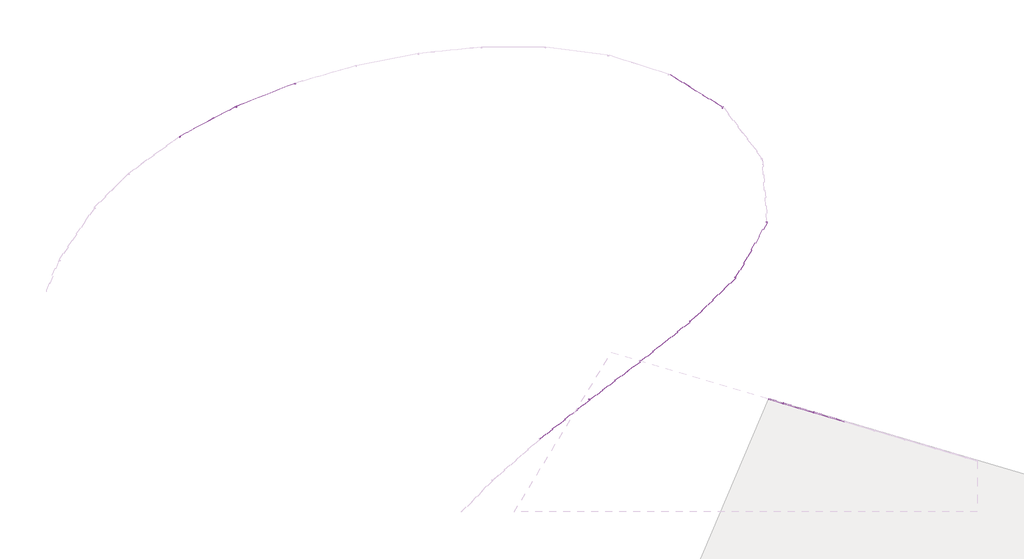
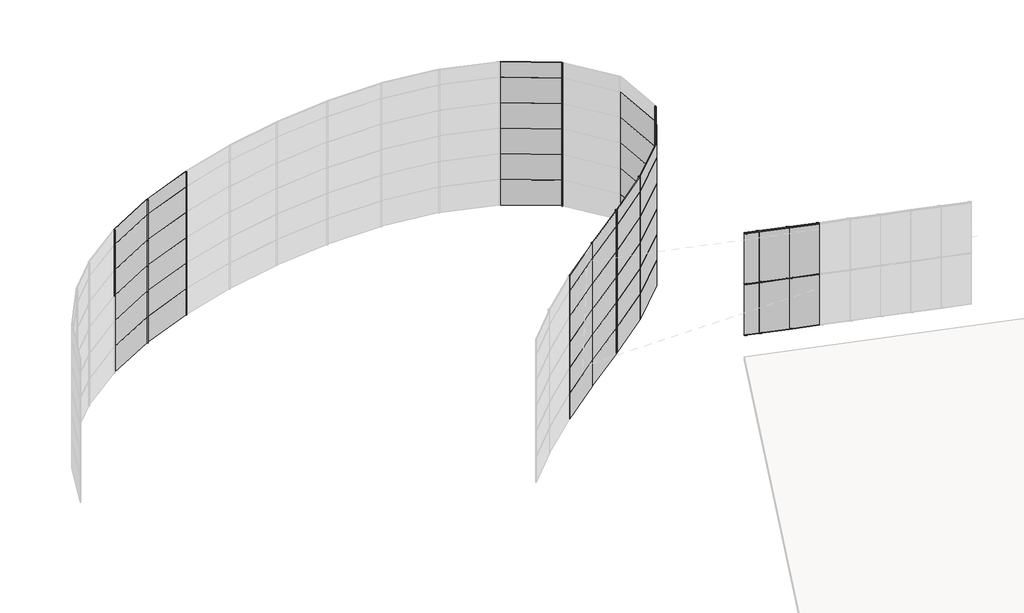
# One storey, part 6 of 8: 60 members, 59 plates.
"""IFC4 building model written with IfcOpenShell, lengths in millimetres."""

import ifcopenshell
import ifcopenshell.guid

model = None  # the IFC model being written
_history = None  # IfcOwnerHistory: only IFC2X3 demands one
_inside = {}  # id of a spatial element -> (the spatial element, [elements in it])
_under = {}  # id of a project, library or spatial element -> (it, [spatial elements below it])
_declared = {}  # id of a project -> (the project, [libraries it declares])
_typed = {}  # id of a type object -> (the type object, [elements of that type])
_made_of = {}  # id of a material, layer set ... -> (it, [elements and type objects made of it])


def new_model(schema):
    """Start an empty IFC model of exactly this schema.

    Asked for "IFC4X3", IfcOpenShell would pick the latest addendum, in which some entities
    have other attributes; the version numbers below select the first issue.
    IFC2X3 requires an IfcOwnerHistory on every rooted entity: one is made here for all.
    """
    global model, _history
    if schema == "IFC4X3":
        model = ifcopenshell.file(schema_version=(4, 3, 0, 0))
    else:
        model = ifcopenshell.file(schema=schema)
    _inside.clear()
    _under.clear()
    _declared.clear()
    _typed.clear()
    _made_of.clear()
    _history = None
    if model.schema == "IFC2X3":
        org = make("IfcOrganization", Name="unknown")
        user = make(
            "IfcPersonAndOrganization",
            ThePerson=make("IfcPerson", FamilyName="unknown"),
            TheOrganization=org,
        )
        app = make(
            "IfcApplication",
            ApplicationDeveloper=org,
            Version="unknown",
            ApplicationFullName="unknown",
            ApplicationIdentifier="unknown",
        )
        _history = make(
            "IfcOwnerHistory",
            OwningUser=user,
            OwningApplication=app,
            ChangeAction="ADDED",
            CreationDate=0,
        )
    return model


def make(cls, **values):
    """One entity of the class cls with the attributes given. An attribute that is None is left unset."""
    return model.create_entity(
        cls, **{name: value for name, value in values.items() if value is not None}
    )


def rooted(cls, **values):
    """An entity with a GlobalId (a new one), such as an element, a storey or a relation."""
    return make(cls, GlobalId=ifcopenshell.guid.new(), OwnerHistory=_history, **values)


def si_unit(unit_type, name, prefix=None):
    """IfcSIUnit, for example si_unit("LENGTHUNIT", "METRE", prefix="MILLI")."""
    return make("IfcSIUnit", UnitType=unit_type, Prefix=prefix, Name=name)


def assignment(units):
    """IfcUnitAssignment: the units of a project."""
    return None if units is None else make("IfcUnitAssignment", Units=units)


def point(xyz):
    """IfcCartesianPoint."""
    return None if xyz is None else make("IfcCartesianPoint", Coordinates=xyz)


def direction(xyz):
    """IfcDirection."""
    return None if xyz is None else make("IfcDirection", DirectionRatios=xyz)


def frame(location, z_axis=None, x_axis=None):
    """IfcAxis2Placement3D, a coordinate frame: its origin and axes. An axis left out is left unset."""
    return make(
        "IfcAxis2Placement3D",
        Location=point(location),
        Axis=direction(z_axis),
        RefDirection=direction(x_axis),
    )


def frame_2d(location, x_axis=None):
    """IfcAxis2Placement2D, a coordinate frame in the plane: its origin and x axis."""
    return make(
        "IfcAxis2Placement2D", Location=point(location), RefDirection=direction(x_axis)
    )


def origin():
    """The frame at (0, 0, 0) with its axes left unset."""
    return frame((0.0, 0.0, 0.0))


def origin_with_axes():
    """The frame at (0, 0, 0) with the z axis (0, 0, 1) and the x axis (1, 0, 0) written out."""
    return frame((0.0, 0.0, 0.0), z_axis=(0.0, 0.0, 1.0), x_axis=(1.0, 0.0, 0.0))


def origin_2d():
    """The frame at (0, 0) in the plane with its x axis left unset."""
    return frame_2d((0.0, 0.0))


def place(relative_to, where):
    """IfcLocalPlacement: puts the frame where relative to a parent placement (None: the world)."""
    return make(
        "IfcLocalPlacement", PlacementRelTo=relative_to, RelativePlacement=where
    )


def context(
    kind, dimensions, precision=None, world=None, true_north=None, identifier=None
):
    """IfcGeometricRepresentationContext, for example the 3D "Model" context."""
    return make(
        "IfcGeometricRepresentationContext",
        ContextIdentifier=identifier,
        ContextType=kind,
        CoordinateSpaceDimension=dimensions,
        Precision=precision,
        WorldCoordinateSystem=world,
        TrueNorth=true_north,
    )


def project(units=None, contexts=None):
    """IfcProject with its units and contexts."""
    return rooted(
        "IfcProject",
        Name="project",
        RepresentationContexts=contexts,
        UnitsInContext=assignment(units),
    )


def spatial(cls, under=None, at=None, **own):
    """A site, building, storey or space (cls), placed at a placement, below another one or the project."""
    s = rooted(cls, ObjectPlacement=at, **own)
    if under is not None:
        _under.setdefault(under.id(), (under, []))[1].append(s)
    return s


def polyline(points):
    """IfcPolyline through the points."""
    return make("IfcPolyline", Points=[point(p) for p in points])


def circle_curve(where, radius):
    """IfcCircle in the frame where."""
    return make("IfcCircle", Position=where, Radius=radius)


def trimmed(basis, trim1, trim2, sense, master):
    """IfcTrimmedCurve: the piece of a basis curve between two trims."""
    return make(
        "IfcTrimmedCurve",
        BasisCurve=basis,
        Trim1=trim1,
        Trim2=trim2,
        SenseAgreement=sense,
        MasterRepresentation=master,
    )


def segment(curve, same_sense, transition):
    """IfcCompositeCurveSegment."""
    return make(
        "IfcCompositeCurveSegment",
        Transition=transition,
        SameSense=same_sense,
        ParentCurve=curve,
    )


def composite_curve(segments, self_intersect=None):
    """IfcCompositeCurve: segments joined end to end."""
    return make("IfcCompositeCurve", Segments=segments, SelfIntersect=self_intersect)


def outline(outer, holes=None, kind="AREA"):
    """IfcArbitraryClosedProfileDef: a profile drawn as a closed curve; with holes, ...WithVoids."""
    if holes is None:
        return make("IfcArbitraryClosedProfileDef", ProfileType=kind, OuterCurve=outer)
    return make(
        "IfcArbitraryProfileDefWithVoids",
        ProfileType=kind,
        OuterCurve=outer,
        InnerCurves=holes,
    )


def extrude(swept, where, along, depth):
    """IfcExtrudedAreaSolid: the profile swept, set in the frame where, extruded along a direction by depth."""
    return make(
        "IfcExtrudedAreaSolid",
        SweptArea=swept,
        Position=where,
        ExtrudedDirection=direction(along),
        Depth=depth,
    )


def shape(context_of_items, identifier, shape_type, items):
    """IfcShapeRepresentation: the items that make up one representation, for example the "Body"."""
    return make(
        "IfcShapeRepresentation",
        ContextOfItems=context_of_items,
        RepresentationIdentifier=identifier,
        RepresentationType=shape_type,
        Items=items,
    )


def source(mapping_origin, context_of_items, identifier, shape_type, items):
    """IfcRepresentationMap: a shape defined once, which mapped items show again and again."""
    return make(
        "IfcRepresentationMap",
        MappingOrigin=mapping_origin,
        MappedRepresentation=shape(context_of_items, identifier, shape_type, items),
    )


def transform(
    local_origin,
    x_axis=None,
    y_axis=None,
    z_axis=None,
    scale=None,
    scale2=None,
    scale3=None,
    uniform=True,
):
    """IfcCartesianTransformationOperator3D, or its non-uniform kind. x_axis, y_axis, z_axis: its Axis1, 2, 3."""
    if uniform:
        return make(
            "IfcCartesianTransformationOperator3D",
            Axis1=direction(x_axis),
            Axis2=direction(y_axis),
            LocalOrigin=point(local_origin),
            Scale=scale,
            Axis3=direction(z_axis),
        )
    return make(
        "IfcCartesianTransformationOperator3DnonUniform",
        Axis1=direction(x_axis),
        Axis2=direction(y_axis),
        LocalOrigin=point(local_origin),
        Scale=scale,
        Axis3=direction(z_axis),
        Scale2=scale2,
        Scale3=scale3,
    )


def mapped(mapping_source, mapping_target):
    """IfcMappedItem: shows the shape of a source again, moved by a transform."""
    return make(
        "IfcMappedItem", MappingSource=mapping_source, MappingTarget=mapping_target
    )


def made_of(thing, what):
    """Note that an element or type object is made of a material, layer set ...; save() writes the relation."""
    if what is not None:
        _made_of.setdefault(what.id(), (what, []))[1].append(thing)
    return thing


def element(
    cls,
    number,
    at=None,
    inside=None,
    cuts=None,
    type_object=None,
    material=None,
    context=None,
    identifier="Body",
    shape_type=None,
    held_by="IfcProductDefinitionShape",
    body=None,
    shapes=None,
    **own,
):
    """One element of the class cls, such as IfcWall. Its Tag is "e" and its number.

    at: its placement. inside: the storey or other place that contains it. cuts: it is an
    opening in that element (IfcRelVoidsElement). A single representation is given by context,
    identifier, shape_type and body (its items); several are given by shapes. held_by: the class
    of the entity that holds the representations. save() writes the other relations.
    """
    e = rooted(cls, Tag="e%d" % number, ObjectPlacement=at, **own)
    if body is not None:
        shapes = [shape(context, identifier, shape_type, body)]
    if shapes is not None:
        e.Representation = make(held_by, Representations=shapes)
    if inside is not None:
        _inside.setdefault(inside.id(), (inside, []))[1].append(e)
    if cuts is not None:
        rooted(
            "IfcRelVoidsElement", RelatingBuildingElement=cuts, RelatedOpeningElement=e
        )
    if type_object is not None:
        _typed.setdefault(type_object.id(), (type_object, []))[1].append(e)
    return made_of(e, material)


def aggregate(whole, parts):
    """IfcRelAggregates: a whole, such as a stair, and the parts it consists of."""
    return rooted("IfcRelAggregates", RelatingObject=whole, RelatedObjects=parts)


def save(model, path):
    """Write the relations noted so far, then the file.

    IfcRelAggregates (storeys below a building ...), IfcRelContainedInSpatialStructure (elements
    in a storey), IfcRelDefinesByType, IfcRelAssociatesMaterial and IfcRelDeclares: one each for
    every whole, place, type object, material and project.
    """
    for whole, parts in _under.values():
        aggregate(whole, parts)
    for where, things in _inside.values():
        rooted(
            "IfcRelContainedInSpatialStructure",
            RelatedElements=things,
            RelatingStructure=where,
        )
    for kind, things in _typed.values():
        rooted("IfcRelDefinesByType", RelatedObjects=things, RelatingType=kind)
    for what, things in _made_of.values():
        rooted("IfcRelAssociatesMaterial", RelatedObjects=things, RelatingMaterial=what)
    for by, libraries in _declared.values():
        rooted("IfcRelDeclares", RelatingContext=by, RelatedDefinitions=libraries)
    model.write(path)


def montante_circular_25_mm_raio_ce826986(model_context):
    return source(origin(), model_context, "Body", "SweptSolid", [
        extrude(outline(composite_curve([segment(trimmed(circle_curve(frame_2d((-25.0, 0.0)), 25.0), [point((0.0, 0.0))], [point((-50.0, 0.0))], False, "CARTESIAN"), True, "CONTINUOUS"), segment(trimmed(circle_curve(frame_2d((-25.0, 0.0)), 25.0), [point((-50.0, 0.0))], [point((0.0, 0.0))], False, "CARTESIAN"), True, "CONTINUOUS")], self_intersect=False)), frame((0.0, 0.0, -1500.0), z_axis=(0.0, 0.0, 1.0), x_axis=(1.0, 0.0, 0.0)), (0.0, 0.0, 1.0), 1500.0),
    ])


def montante_circular_25_mm_raio_36e581cf(model_context):
    return source(origin(), model_context, "Body", "SweptSolid", [
        extrude(outline(composite_curve([segment(trimmed(circle_curve(origin_2d(), 25.0), [point((25.0, 0.0))], [point((-25.0, 0.0))], False, "CARTESIAN"), True, "CONTINUOUS"), segment(trimmed(circle_curve(origin_2d(), 25.0), [point((-25.0, 0.0))], [point((25.0, 0.0))], False, "CARTESIAN"), True, "CONTINUOUS")], self_intersect=False)), frame((0.0, 0.0, -1500.0), z_axis=(0.0, 0.0, 1.0), x_axis=(1.0, 0.0, 0.0)), (0.0, 0.0, 1.0), 1500.0),
    ])


def montante_circular_25_mm_raio_f24612f6(model_context):
    return source(origin(), model_context, "Body", "SweptSolid", [
        extrude(outline(composite_curve([segment(trimmed(circle_curve(frame_2d((-25.0, 0.0)), 25.0), [point((0.0, 0.0))], [point((-50.0, 0.0))], False, "CARTESIAN"), True, "CONTINUOUS"), segment(trimmed(circle_curve(frame_2d((-25.0, 0.0)), 25.0), [point((-50.0, 0.0))], [point((0.0, 0.0))], False, "CARTESIAN"), True, "CONTINUOUS")], self_intersect=False)), frame((0.0, 0.0, -727.4383788), z_axis=(0.0, 0.0, 1.0), x_axis=(1.0, 0.0, 0.0)), (0.0, 0.0, 1.0), 727.4383788),
    ])


def montante_circular_25_mm_raio_a1f35a82(model_context):
    return source(origin(), model_context, "Body", "SweptSolid", [
        extrude(outline(composite_curve([segment(trimmed(circle_curve(origin_2d(), 25.0), [point((25.0, 0.0))], [point((-25.0, 0.0))], False, "CARTESIAN"), True, "CONTINUOUS"), segment(trimmed(circle_curve(origin_2d(), 25.0), [point((-25.0, 0.0))], [point((25.0, 0.0))], False, "CARTESIAN"), True, "CONTINUOUS")], self_intersect=False)), frame((0.0, 0.0, -727.4383788), z_axis=(0.0, 0.0, 1.0), x_axis=(1.0, 0.0, 0.0)), (0.0, 0.0, 1.0), 727.4383788),
    ])


def montante_circular_25_mm_raio_8ba79aec(model_context):
    return source(origin(), model_context, "Body", "SweptSolid", [
        extrude(outline(composite_curve([segment(trimmed(circle_curve(origin_2d(), 25.0), [point((25.0, 0.0))], [point((-25.0, 0.0))], False, "CARTESIAN"), True, "CONTINUOUS"), segment(trimmed(circle_curve(origin_2d(), 25.0), [point((-25.0, 0.0))], [point((25.0, 0.0))], False, "CARTESIAN"), True, "CONTINUOUS")], self_intersect=False)), frame((0.0, 0.0, -900.0), z_axis=(0.0, 0.0, 1.0), x_axis=(1.0, 0.0, 0.0)), (0.0, 0.0, 1.0), 900.0),
    ])


def painel_do_sistema_5ef9eced(model_context):
    return source(origin(), model_context, "Body", "SweptSolid", [
        extrude(outline(polyline([(1475.0, 24.5), (-1475.0, 24.5), (-1475.0, 49.5), (1475.0, 49.5), (1475.0, 24.5)])), origin_with_axes(), (0.0, 0.0, 1.0), 1500.0),
    ])


def painel_do_sistema_bf426e09(model_context):
    return source(origin(), model_context, "Body", "SweptSolid", [
        extrude(outline(polyline([(1475.0, 24.5), (-1475.0, 24.5), (-1475.0, 49.5), (1475.0, 49.5), (1475.0, 24.5)])), origin_with_axes(), (0.0, 0.0, 1.0), 727.4383788),
    ])


def painel_do_sistema_85ccde5d(model_context):
    return source(origin(), model_context, "Body", "SweptSolid", [
        extrude(outline(polyline([(1475.0, -49.5), (-1475.0, -49.5), (-1475.0, -24.5), (1475.0, -24.5), (1475.0, -49.5)])), origin_with_axes(), (0.0, 0.0, 1.0), 1500.0),
    ])


def painel_do_sistema_d8fd150b(model_context):
    return source(origin(), model_context, "Body", "SweptSolid", [
        extrude(outline(polyline([(1475.0, -49.5), (-1475.0, -49.5), (-1475.0, -24.5), (1475.0, -24.5), (1475.0, -49.5)])), origin_with_axes(), (0.0, 0.0, 1.0), 900.0),
    ])


def painel_do_sistema_af596b93(model_context):
    return source(origin(), model_context, "Body", "SweptSolid", [
        extrude(outline(polyline([(1462.4999925, 24.5), (-1462.4999925, 24.5), (-1462.4999925, 49.5), (1462.4999925, 49.5), (1462.4999925, 24.5)])), origin_with_axes(), (0.0, 0.0, 1.0), 1500.0),
    ])


def painel_do_sistema_44dfe8f0(model_context):
    return source(origin(), model_context, "Body", "SweptSolid", [
        extrude(outline(polyline([(1462.4999925, 24.5), (-1462.4999925, 24.5), (-1462.4999925, 49.5), (1462.4999925, 49.5), (1462.4999925, 24.5)])), origin_with_axes(), (0.0, 0.0, 1.0), 727.4383788),
    ])


model = new_model("IFC4")

# Units and contexts
model_context = context("Model", 3, world=origin())
ifc_project = project(units=[si_unit("LENGTHUNIT", "METRE", prefix="MILLI")], contexts=[model_context])

# Site, building, storey
site = spatial("IfcSite", under=ifc_project)
building = spatial("IfcBuilding", under=site)
storey = spatial("IfcBuildingStorey", under=building, Name="Nível 3", Elevation=7695.2)

# Members
placement = place(None, origin())
montante_circular_25_mm_raio_shape = montante_circular_25_mm_raio_ce826986(model_context)
element("IfcMember", 1, ObjectType="Montante circular : 25 mm Raio", at=placement, inside=storey, context=model_context, shape_type="MappedRepresentation", body=[
    mapped(montante_circular_25_mm_raio_shape, transform((-4389.7681283, 32366.1480949, 15000.0), x_axis=(0.0, 0.0, 1.0), y_axis=(0.28318378939534594, 0.95906566064253, 0.0), z_axis=(-0.95906566064253, 0.28318378939534594, 0.0))),
])
element("IfcMember", 2, ObjectType="Montante circular : 25 mm Raio", at=placement, inside=storey, context=model_context, shape_type="MappedRepresentation", body=[
    mapped(montante_circular_25_mm_raio_shape, transform((-5828.3666192, 32790.923779, 15000.0), x_axis=(0.0, 0.0, 1.0), y_axis=(0.283183789395347, 0.9590656606425296, 0.0), z_axis=(-0.9590656606425296, 0.283183789395347, 0.0))),
])
montante_circular_25_mm_raio_2_shape = montante_circular_25_mm_raio_36e581cf(model_context)
element("IfcMember", 3, ObjectType="Montante circular : 25 mm Raio", at=placement, inside=storey, context=model_context, shape_type="MappedRepresentation", body=[
    mapped(montante_circular_25_mm_raio_2_shape, transform((-4389.7681283, 32366.1480949, 9000.000015), x_axis=(0.0, 0.0, 1.0), y_axis=(0.28318378939534594, 0.95906566064253, 0.0), z_axis=(-0.95906566064253, 0.28318378939534594, 0.0))),
])
element("IfcMember", 4, ObjectType="Montante circular : 25 mm Raio", at=placement, inside=storey, context=model_context, shape_type="MappedRepresentation", body=[
    mapped(montante_circular_25_mm_raio_2_shape, transform((-5828.3666192, 32790.923779, 9000.000015), x_axis=(0.0, 0.0, 1.0), y_axis=(0.283183789395347, 0.9590656606425296, 0.0), z_axis=(-0.9590656606425296, 0.283183789395347, 0.0))),
])
element("IfcMember", 5, ObjectType="Montante circular : 25 mm Raio", at=placement, inside=storey, context=model_context, shape_type="MappedRepresentation", body=[
    mapped(montante_circular_25_mm_raio_2_shape, transform((-4389.7681283, 32366.1480949, 12000.000015), x_axis=(0.0, 0.0, 1.0), y_axis=(0.28318378939534855, 0.9590656606425292, 0.0), z_axis=(-0.9590656606425291, 0.2831837893953485, 0.0))),
])
element("IfcMember", 6, ObjectType="Montante circular : 25 mm Raio", at=placement, inside=storey, context=model_context, shape_type="MappedRepresentation", body=[
    mapped(montante_circular_25_mm_raio_2_shape, transform((-5828.3666192, 32790.923779, 12000.000015), x_axis=(0.0, 0.0, 1.0), y_axis=(0.283183789395347, 0.9590656606425296, 0.0), z_axis=(-0.9590656606425296, 0.283183789395347, 0.0))),
])
element("IfcMember", 7, ObjectType="Montante circular : 25 mm Raio", at=placement, inside=storey, context=model_context, shape_type="MappedRepresentation", body=[
    mapped(montante_circular_25_mm_raio_2_shape, transform((-14996.1891623, 32974.6356945, 9000.0), x_axis=(0.7952150611070873, 0.6063274747102028, 0.0), y_axis=(0.6063274747102028, -0.7952150611070873, 0.0), z_axis=(0.0, 0.0, -1.0))),
])
element("IfcMember", 8, ObjectType="Montante circular : 25 mm Raio", at=placement, inside=storey, context=model_context, shape_type="MappedRepresentation", body=[
    mapped(montante_circular_25_mm_raio_2_shape, transform((-12604.1298635, 34785.1749266, 9000.0), x_axis=(0.7953870623365296, 0.6061018240095187, 0.0), y_axis=(0.6061018240095187, -0.7953870623365296, 0.0), z_axis=(0.0, 0.0, -1.0))),
])
element("IfcMember", 9, ObjectType="Montante circular : 25 mm Raio", at=placement, inside=storey, context=model_context, shape_type="MappedRepresentation", body=[
    mapped(montante_circular_25_mm_raio_2_shape, transform((-10255.474771, 36651.6741247, 9000.0), x_axis=(0.7627263023971693, 0.6467214142361005, 0.0), y_axis=(0.6467214142361005, -0.7627263023971693, 0.0), z_axis=(0.0, 0.0, -1.0))),
])
element("IfcMember", 10, ObjectType="Montante circular : 25 mm Raio", at=placement, inside=storey, context=model_context, shape_type="MappedRepresentation", body=[
    mapped(montante_circular_25_mm_raio_2_shape, transform((-8101.871437, 38740.2125323, 9000.0), x_axis=(0.6490334571140042, 0.7607598645739956, 0.0), y_axis=(0.7607598645739956, -0.6490334571140042, 0.0), z_axis=(0.0, 0.0, -1.0))),
])
element("IfcMember", 11, ObjectType="Montante circular : 25 mm Raio", at=placement, inside=storey, context=model_context, shape_type="MappedRepresentation", body=[
    mapped(montante_circular_25_mm_raio_2_shape, transform((-6627.5874319, 41352.9671461, 9000.0), x_axis=(0.24827563424230142, 0.9686894287859154, 0.0), y_axis=(0.9686894287859154, -0.24827563424230142, 0.0), z_axis=(0.0, 0.0, -1.0))),
])
element("IfcMember", 12, ObjectType="Montante circular : 25 mm Raio", at=placement, inside=storey, context=model_context, shape_type="MappedRepresentation", body=[
    mapped(montante_circular_25_mm_raio_2_shape, transform((-8685.5307871, 46730.4667655, 9000.0), x_axis=(-0.7608105002607386, 0.6489741001711892, 0.0), y_axis=(0.6489741001711892, 0.7608105002607386, 0.0), z_axis=(0.0, 0.0, -1.0))),
])
element("IfcMember", 13, ObjectType="Montante circular : 25 mm Raio", at=placement, inside=storey, context=model_context, shape_type="MappedRepresentation", body=[
    mapped(montante_circular_25_mm_raio_2_shape, transform((-28892.5410808, 47874.3709699, 9000.0), x_axis=(-0.9471529213375351, -0.3207823929111028, 0.0), y_axis=(-0.3207823929111028, 0.9471529213375351, 0.0), z_axis=(0.0, 0.0, -1.0))),
])
element("IfcMember", 14, ObjectType="Montante circular : 25 mm Raio", at=placement, inside=storey, context=model_context, shape_type="MappedRepresentation", body=[
    mapped(montante_circular_25_mm_raio_2_shape, transform((-31682.4252949, 46771.3994961, 9000.0), x_axis=(-0.9093535544571357, -0.4160241735718888, 0.0), y_axis=(-0.4160241735718888, 0.9093535544571357, 0.0), z_axis=(0.0, 0.0, -1.0))),
])
element("IfcMember", 15, ObjectType="Montante circular : 25 mm Raio", at=placement, inside=storey, context=model_context, shape_type="MappedRepresentation", body=[
    mapped(montante_circular_25_mm_raio_2_shape, transform((-14996.1891623, 32974.6356945, 10500.0), x_axis=(0.7952150611070873, 0.6063274747102028, 0.0), y_axis=(0.6063274747102028, -0.7952150611070873, 0.0), z_axis=(0.0, 0.0, -1.0))),
])
element("IfcMember", 16, ObjectType="Montante circular : 25 mm Raio", at=placement, inside=storey, context=model_context, shape_type="MappedRepresentation", body=[
    mapped(montante_circular_25_mm_raio_2_shape, transform((-12604.1298635, 34785.1749266, 10500.0), x_axis=(0.7953870623365298, 0.6061018240095186, 0.0), y_axis=(0.6061018240095186, -0.7953870623365298, 0.0), z_axis=(0.0, 0.0, -1.0))),
])
element("IfcMember", 17, ObjectType="Montante circular : 25 mm Raio", at=placement, inside=storey, context=model_context, shape_type="MappedRepresentation", body=[
    mapped(montante_circular_25_mm_raio_2_shape, transform((-10255.474771, 36651.6741247, 10500.0), x_axis=(0.7627263023971693, 0.6467214142361005, 0.0), y_axis=(0.6467214142361005, -0.7627263023971693, 0.0), z_axis=(0.0, 0.0, -1.0))),
])
element("IfcMember", 18, ObjectType="Montante circular : 25 mm Raio", at=placement, inside=storey, context=model_context, shape_type="MappedRepresentation", body=[
    mapped(montante_circular_25_mm_raio_2_shape, transform((-8101.871437, 38740.2125323, 10500.0), x_axis=(0.6490334571140042, 0.7607598645739956, 0.0), y_axis=(0.7607598645739956, -0.6490334571140042, 0.0), z_axis=(0.0, 0.0, -1.0))),
])
element("IfcMember", 19, ObjectType="Montante circular : 25 mm Raio", at=placement, inside=storey, context=model_context, shape_type="MappedRepresentation", body=[
    mapped(montante_circular_25_mm_raio_2_shape, transform((-6627.5874319, 41352.9671461, 10500.0), x_axis=(0.24827563424230142, 0.9686894287859154, 0.0), y_axis=(0.9686894287859154, -0.24827563424230142, 0.0), z_axis=(0.0, 0.0, -1.0))),
])
element("IfcMember", 20, ObjectType="Montante circular : 25 mm Raio", at=placement, inside=storey, context=model_context, shape_type="MappedRepresentation", body=[
    mapped(montante_circular_25_mm_raio_2_shape, transform((-8685.5307871, 46730.4667655, 10500.0), x_axis=(-0.7608105002607386, 0.6489741001711892, 0.0), y_axis=(0.6489741001711892, 0.7608105002607386, 0.0), z_axis=(0.0, 0.0, -1.0))),
])
element("IfcMember", 21, ObjectType="Montante circular : 25 mm Raio", at=placement, inside=storey, context=model_context, shape_type="MappedRepresentation", body=[
    mapped(montante_circular_25_mm_raio_2_shape, transform((-28892.5410808, 47874.3709699, 10500.0), x_axis=(-0.9471529213375351, -0.3207823929111028, 0.0), y_axis=(-0.3207823929111028, 0.9471529213375351, 0.0), z_axis=(0.0, 0.0, -1.0))),
])
element("IfcMember", 22, ObjectType="Montante circular : 25 mm Raio", at=placement, inside=storey, context=model_context, shape_type="MappedRepresentation", body=[
    mapped(montante_circular_25_mm_raio_2_shape, transform((-31682.4252949, 46771.3994961, 10500.0), x_axis=(-0.9093535544571357, -0.4160241735718888, 0.0), y_axis=(-0.4160241735718888, 0.9093535544571357, 0.0), z_axis=(0.0, 0.0, -1.0))),
])
element("IfcMember", 23, ObjectType="Montante circular : 25 mm Raio", at=placement, inside=storey, context=model_context, shape_type="MappedRepresentation", body=[
    mapped(montante_circular_25_mm_raio_2_shape, transform((-14996.1891623, 32974.6356945, 12000.0), x_axis=(0.7952150611070873, 0.6063274747102027, 0.0), y_axis=(0.6063274747102027, -0.7952150611070873, 0.0), z_axis=(0.0, 0.0, -1.0))),
])
element("IfcMember", 24, ObjectType="Montante circular : 25 mm Raio", at=placement, inside=storey, context=model_context, shape_type="MappedRepresentation", body=[
    mapped(montante_circular_25_mm_raio_2_shape, transform((-12604.1298635, 34785.1749266, 12000.0), x_axis=(0.7953870623365298, 0.6061018240095186, 0.0), y_axis=(0.6061018240095186, -0.7953870623365298, 0.0), z_axis=(0.0, 0.0, -1.0))),
])
element("IfcMember", 25, ObjectType="Montante circular : 25 mm Raio", at=placement, inside=storey, context=model_context, shape_type="MappedRepresentation", body=[
    mapped(montante_circular_25_mm_raio_2_shape, transform((-10255.474771, 36651.6741247, 12000.0), x_axis=(0.7627263023971693, 0.6467214142361005, 0.0), y_axis=(0.6467214142361005, -0.7627263023971693, 0.0), z_axis=(0.0, 0.0, -1.0))),
])
element("IfcMember", 26, ObjectType="Montante circular : 25 mm Raio", at=placement, inside=storey, context=model_context, shape_type="MappedRepresentation", body=[
    mapped(montante_circular_25_mm_raio_2_shape, transform((-8101.871437, 38740.2125323, 12000.0), x_axis=(0.6490334571140043, 0.7607598645739955, 0.0), y_axis=(0.7607598645739955, -0.6490334571140043, 0.0), z_axis=(0.0, 0.0, -1.0))),
])
element("IfcMember", 27, ObjectType="Montante circular : 25 mm Raio", at=placement, inside=storey, context=model_context, shape_type="MappedRepresentation", body=[
    mapped(montante_circular_25_mm_raio_2_shape, transform((-6627.5874319, 41352.9671461, 12000.0), x_axis=(0.24827563424230145, 0.9686894287859155, 0.0), y_axis=(0.9686894287859155, -0.24827563424230145, 0.0), z_axis=(0.0, 0.0, -1.0))),
])
element("IfcMember", 28, ObjectType="Montante circular : 25 mm Raio", at=placement, inside=storey, context=model_context, shape_type="MappedRepresentation", body=[
    mapped(montante_circular_25_mm_raio_2_shape, transform((-8685.5307871, 46730.4667655, 12000.0), x_axis=(-0.7608105002607383, 0.6489741001711896, 0.0), y_axis=(0.6489741001711896, 0.7608105002607383, 0.0), z_axis=(0.0, 0.0, -1.0))),
])
element("IfcMember", 29, ObjectType="Montante circular : 25 mm Raio", at=placement, inside=storey, context=model_context, shape_type="MappedRepresentation", body=[
    mapped(montante_circular_25_mm_raio_2_shape, transform((-28892.5410808, 47874.3709699, 12000.0), x_axis=(-0.9471529213375351, -0.3207823929111028, 0.0), y_axis=(-0.3207823929111028, 0.9471529213375351, 0.0), z_axis=(0.0, 0.0, -1.0))),
])
element("IfcMember", 30, ObjectType="Montante circular : 25 mm Raio", at=placement, inside=storey, context=model_context, shape_type="MappedRepresentation", body=[
    mapped(montante_circular_25_mm_raio_2_shape, transform((-31682.4252949, 46771.3994961, 12000.0), x_axis=(-0.9093535544571357, -0.4160241735718888, 0.0), y_axis=(-0.4160241735718888, 0.9093535544571357, 0.0), z_axis=(0.0, 0.0, -1.0))),
])
element("IfcMember", 31, ObjectType="Montante circular : 25 mm Raio", at=placement, inside=storey, context=model_context, shape_type="MappedRepresentation", body=[
    mapped(montante_circular_25_mm_raio_2_shape, transform((-14996.1891623, 32974.6356945, 13500.0), x_axis=(0.7952150611070873, 0.6063274747102028, 0.0), y_axis=(0.6063274747102028, -0.7952150611070873, 0.0), z_axis=(0.0, 0.0, -1.0))),
])
element("IfcMember", 32, ObjectType="Montante circular : 25 mm Raio", at=placement, inside=storey, context=model_context, shape_type="MappedRepresentation", body=[
    mapped(montante_circular_25_mm_raio_2_shape, transform((-12604.1298635, 34785.1749266, 13500.0), x_axis=(0.7953870623365296, 0.6061018240095187, 0.0), y_axis=(0.6061018240095187, -0.7953870623365296, 0.0), z_axis=(0.0, 0.0, -1.0))),
])
element("IfcMember", 33, ObjectType="Montante circular : 25 mm Raio", at=placement, inside=storey, context=model_context, shape_type="MappedRepresentation", body=[
    mapped(montante_circular_25_mm_raio_2_shape, transform((-10255.474771, 36651.6741247, 13500.0), x_axis=(0.7627263023971693, 0.6467214142361005, 0.0), y_axis=(0.6467214142361005, -0.7627263023971693, 0.0), z_axis=(0.0, 0.0, -1.0))),
])
element("IfcMember", 34, ObjectType="Montante circular : 25 mm Raio", at=placement, inside=storey, context=model_context, shape_type="MappedRepresentation", body=[
    mapped(montante_circular_25_mm_raio_2_shape, transform((-8101.871437, 38740.2125323, 13500.0), x_axis=(0.6490334571140042, 0.7607598645739956, 0.0), y_axis=(0.7607598645739956, -0.6490334571140042, 0.0), z_axis=(0.0, 0.0, -1.0))),
])
element("IfcMember", 35, ObjectType="Montante circular : 25 mm Raio", at=placement, inside=storey, context=model_context, shape_type="MappedRepresentation", body=[
    mapped(montante_circular_25_mm_raio_2_shape, transform((-6627.5874319, 41352.9671461, 13500.0), x_axis=(0.24827563424230142, 0.9686894287859154, 0.0), y_axis=(0.9686894287859154, -0.24827563424230142, 0.0), z_axis=(0.0, 0.0, -1.0))),
])
element("IfcMember", 36, ObjectType="Montante circular : 25 mm Raio", at=placement, inside=storey, context=model_context, shape_type="MappedRepresentation", body=[
    mapped(montante_circular_25_mm_raio_2_shape, transform((-8685.5307871, 46730.4667655, 13500.0), x_axis=(-0.7608105002607386, 0.6489741001711892, 0.0), y_axis=(0.6489741001711892, 0.7608105002607386, 0.0), z_axis=(0.0, 0.0, -1.0))),
])
element("IfcMember", 37, ObjectType="Montante circular : 25 mm Raio", at=placement, inside=storey, context=model_context, shape_type="MappedRepresentation", body=[
    mapped(montante_circular_25_mm_raio_2_shape, transform((-28892.5410808, 47874.3709699, 13500.0), x_axis=(-0.9471529213375351, -0.3207823929111028, 0.0), y_axis=(-0.3207823929111028, 0.9471529213375351, 0.0), z_axis=(0.0, 0.0, -1.0))),
])
element("IfcMember", 38, ObjectType="Montante circular : 25 mm Raio", at=placement, inside=storey, context=model_context, shape_type="MappedRepresentation", body=[
    mapped(montante_circular_25_mm_raio_2_shape, transform((-31682.4252949, 46771.3994961, 13500.0), x_axis=(-0.9093535544571357, -0.4160241735718888, 0.0), y_axis=(-0.4160241735718888, 0.9093535544571357, 0.0), z_axis=(0.0, 0.0, -1.0))),
])
element("IfcMember", 39, ObjectType="Montante circular : 25 mm Raio", at=placement, inside=storey, context=model_context, shape_type="MappedRepresentation", body=[
    mapped(montante_circular_25_mm_raio_2_shape, transform((-34331.1697585, 45362.7999198, 13500.0), x_axis=(-0.850927589483555, -0.5252830070121313, 0.0), y_axis=(-0.5252830070121313, 0.850927589483555, 0.0), z_axis=(0.0, 0.0, -1.0))),
])
element("IfcMember", 40, ObjectType="Montante circular : 25 mm Raio", at=placement, inside=storey, context=model_context, shape_type="MappedRepresentation", body=[
    mapped(montante_circular_25_mm_raio_2_shape, transform((-14996.1891623, 32974.6356945, 15000.0), x_axis=(0.7952150611070873, 0.6063274747102028, 0.0), y_axis=(0.6063274747102028, -0.7952150611070873, 0.0), z_axis=(0.0, 0.0, -1.0))),
])
element("IfcMember", 41, ObjectType="Montante circular : 25 mm Raio", at=placement, inside=storey, context=model_context, shape_type="MappedRepresentation", body=[
    mapped(montante_circular_25_mm_raio_2_shape, transform((-12604.1298635, 34785.1749266, 15000.0), x_axis=(0.7953870623365296, 0.6061018240095187, 0.0), y_axis=(0.6061018240095187, -0.7953870623365296, 0.0), z_axis=(0.0, 0.0, -1.0))),
])
element("IfcMember", 42, ObjectType="Montante circular : 25 mm Raio", at=placement, inside=storey, context=model_context, shape_type="MappedRepresentation", body=[
    mapped(montante_circular_25_mm_raio_2_shape, transform((-10255.474771, 36651.6741247, 15000.0), x_axis=(0.7627263023971693, 0.6467214142361005, 0.0), y_axis=(0.6467214142361005, -0.7627263023971693, 0.0), z_axis=(0.0, 0.0, -1.0))),
])
element("IfcMember", 43, ObjectType="Montante circular : 25 mm Raio", at=placement, inside=storey, context=model_context, shape_type="MappedRepresentation", body=[
    mapped(montante_circular_25_mm_raio_2_shape, transform((-8101.871437, 38740.2125323, 15000.0), x_axis=(0.6490334571140042, 0.7607598645739956, 0.0), y_axis=(0.7607598645739956, -0.6490334571140042, 0.0), z_axis=(0.0, 0.0, -1.0))),
])
element("IfcMember", 44, ObjectType="Montante circular : 25 mm Raio", at=placement, inside=storey, context=model_context, shape_type="MappedRepresentation", body=[
    mapped(montante_circular_25_mm_raio_2_shape, transform((-6627.5874319, 41352.9671461, 15000.0), x_axis=(0.24827563424230142, 0.9686894287859154, 0.0), y_axis=(0.9686894287859154, -0.24827563424230142, 0.0), z_axis=(0.0, 0.0, -1.0))),
])
element("IfcMember", 45, ObjectType="Montante circular : 25 mm Raio", at=placement, inside=storey, context=model_context, shape_type="MappedRepresentation", body=[
    mapped(montante_circular_25_mm_raio_2_shape, transform((-8685.5307871, 46730.4667655, 15000.0), x_axis=(-0.7608105002607386, 0.6489741001711892, 0.0), y_axis=(0.6489741001711892, 0.7608105002607386, 0.0), z_axis=(0.0, 0.0, -1.0))),
])
element("IfcMember", 46, ObjectType="Montante circular : 25 mm Raio", at=placement, inside=storey, context=model_context, shape_type="MappedRepresentation", body=[
    mapped(montante_circular_25_mm_raio_2_shape, transform((-28892.5410808, 47874.3709699, 15000.0), x_axis=(-0.9471529213375351, -0.3207823929111028, 0.0), y_axis=(-0.3207823929111028, 0.9471529213375351, 0.0), z_axis=(0.0, 0.0, -1.0))),
])
element("IfcMember", 47, ObjectType="Montante circular : 25 mm Raio", at=placement, inside=storey, context=model_context, shape_type="MappedRepresentation", body=[
    mapped(montante_circular_25_mm_raio_2_shape, transform((-31682.4252949, 46771.3994961, 15000.0), x_axis=(-0.9093535544571357, -0.4160241735718888, 0.0), y_axis=(-0.4160241735718888, 0.9093535544571357, 0.0), z_axis=(0.0, 0.0, -1.0))),
])
element("IfcMember", 48, ObjectType="Montante circular : 25 mm Raio", at=placement, inside=storey, context=model_context, shape_type="MappedRepresentation", body=[
    mapped(montante_circular_25_mm_raio_2_shape, transform((-34331.1697585, 45362.7999198, 15000.0), x_axis=(-0.8509275894835548, -0.5252830070121313, 0.0), y_axis=(-0.5252830070121313, 0.8509275894835548, 0.0), z_axis=(0.0, 0.0, -1.0))),
])
montante_circular_25_mm_raio_3_shape = montante_circular_25_mm_raio_f24612f6(model_context)
element("IfcMember", 49, ObjectType="Montante circular : 25 mm Raio", at=placement, inside=storey, context=model_context, shape_type="MappedRepresentation", body=[
    mapped(montante_circular_25_mm_raio_3_shape, transform((-6526.0277886, 32996.9225357, 15000.0), x_axis=(0.0, 0.0, 1.0), y_axis=(0.28318378939534294, 0.9590656606425308, 0.0), z_axis=(-0.9590656606425308, 0.28318378939534294, 0.0))),
])
montante_circular_25_mm_raio_4_shape = montante_circular_25_mm_raio_a1f35a82(model_context)
element("IfcMember", 50, ObjectType="Montante circular : 25 mm Raio", at=placement, inside=storey, context=model_context, shape_type="MappedRepresentation", body=[
    mapped(montante_circular_25_mm_raio_4_shape, transform((-6526.0277886, 32996.9225357, 9000.000015), x_axis=(0.0, 0.0, 1.0), y_axis=(0.28318378939534294, 0.9590656606425308, 0.0), z_axis=(-0.9590656606425308, 0.28318378939534294, 0.0))),
])
element("IfcMember", 51, ObjectType="Montante circular : 25 mm Raio", at=placement, inside=storey, context=model_context, shape_type="MappedRepresentation", body=[
    mapped(montante_circular_25_mm_raio_4_shape, transform((-6526.0277886, 32996.9225357, 12000.000015), x_axis=(0.0, 0.0, 1.0), y_axis=(0.28318378939534294, 0.9590656606425308, 0.0), z_axis=(-0.9590656606425308, 0.28318378939534294, 0.0))),
])
montante_circular_25_mm_raio_5_shape = montante_circular_25_mm_raio_8ba79aec(model_context)
element("IfcMember", 52, ObjectType="Montante circular : 25 mm Raio", at=placement, inside=storey, context=model_context, shape_type="MappedRepresentation", body=[
    mapped(montante_circular_25_mm_raio_5_shape, transform((-14996.1891623, 32974.6356945, 16500.0), x_axis=(0.7952150611070873, 0.6063274747102028, 0.0), y_axis=(0.6063274747102028, -0.7952150611070873, 0.0), z_axis=(0.0, 0.0, -1.0))),
])
element("IfcMember", 53, ObjectType="Montante circular : 25 mm Raio", at=placement, inside=storey, context=model_context, shape_type="MappedRepresentation", body=[
    mapped(montante_circular_25_mm_raio_5_shape, transform((-12604.1298635, 34785.1749266, 16500.0), x_axis=(0.7953870623365296, 0.6061018240095187, 0.0), y_axis=(0.6061018240095187, -0.7953870623365296, 0.0), z_axis=(0.0, 0.0, -1.0))),
])
element("IfcMember", 54, ObjectType="Montante circular : 25 mm Raio", at=placement, inside=storey, context=model_context, shape_type="MappedRepresentation", body=[
    mapped(montante_circular_25_mm_raio_5_shape, transform((-10255.474771, 36651.6741247, 16500.0), x_axis=(0.7627263023971693, 0.6467214142361005, 0.0), y_axis=(0.6467214142361005, -0.7627263023971693, 0.0), z_axis=(0.0, 0.0, -1.0))),
])
element("IfcMember", 55, ObjectType="Montante circular : 25 mm Raio", at=placement, inside=storey, context=model_context, shape_type="MappedRepresentation", body=[
    mapped(montante_circular_25_mm_raio_5_shape, transform((-8101.871437, 38740.2125323, 16500.0), x_axis=(0.6490334571140042, 0.7607598645739956, 0.0), y_axis=(0.7607598645739956, -0.6490334571140042, 0.0), z_axis=(0.0, 0.0, -1.0))),
])
element("IfcMember", 56, ObjectType="Montante circular : 25 mm Raio", at=placement, inside=storey, context=model_context, shape_type="MappedRepresentation", body=[
    mapped(montante_circular_25_mm_raio_5_shape, transform((-6627.5874319, 41352.9671461, 16500.0), x_axis=(0.24827563424230142, 0.9686894287859154, 0.0), y_axis=(0.9686894287859154, -0.24827563424230142, 0.0), z_axis=(0.0, 0.0, -1.0))),
])
element("IfcMember", 57, ObjectType="Montante circular : 25 mm Raio", at=placement, inside=storey, context=model_context, shape_type="MappedRepresentation", body=[
    mapped(montante_circular_25_mm_raio_5_shape, transform((-8685.5307871, 46730.4667655, 16500.0), x_axis=(-0.7608105002607386, 0.6489741001711892, 0.0), y_axis=(0.6489741001711892, 0.7608105002607386, 0.0), z_axis=(0.0, 0.0, -1.0))),
])
element("IfcMember", 58, ObjectType="Montante circular : 25 mm Raio", at=placement, inside=storey, context=model_context, shape_type="MappedRepresentation", body=[
    mapped(montante_circular_25_mm_raio_5_shape, transform((-28892.5410808, 47874.3709699, 16500.0), x_axis=(-0.9471529213375351, -0.3207823929111028, 0.0), y_axis=(-0.3207823929111028, 0.9471529213375351, 0.0), z_axis=(0.0, 0.0, -1.0))),
])
element("IfcMember", 59, ObjectType="Montante circular : 25 mm Raio", at=placement, inside=storey, context=model_context, shape_type="MappedRepresentation", body=[
    mapped(montante_circular_25_mm_raio_5_shape, transform((-31682.4252949, 46771.3994961, 16500.0), x_axis=(-0.9093535544571357, -0.4160241735718888, 0.0), y_axis=(-0.4160241735718888, 0.9093535544571357, 0.0), z_axis=(0.0, 0.0, -1.0))),
])
element("IfcMember", 60, ObjectType="Montante circular : 25 mm Raio", at=placement, inside=storey, context=model_context, shape_type="MappedRepresentation", body=[
    mapped(montante_circular_25_mm_raio_5_shape, transform((-34331.1697585, 45362.7999198, 16500.0), x_axis=(-0.850927589483555, -0.5252830070121313, 0.0), y_axis=(-0.5252830070121313, 0.850927589483555, 0.0), z_axis=(0.0, 0.0, -1.0))),
])

# Plates
painel_do_sistema_shape = painel_do_sistema_5ef9eced(model_context)
element("IfcPlate", 61, ObjectType="Painel do sistema", at=placement, inside=storey, context=model_context, shape_type="MappedRepresentation", body=[
    mapped(painel_do_sistema_shape, transform((-4389.7681283, 32366.1480949, 10500.000015), x_axis=(0.0, 0.0, 1.0), y_axis=(-0.2831837893953486, -0.9590656606425292, 0.0), z_axis=(0.9590656606425292, -0.2831837893953486, 0.0))),
])
element("IfcPlate", 62, ObjectType="Painel do sistema", at=placement, inside=storey, context=model_context, shape_type="MappedRepresentation", body=[
    mapped(painel_do_sistema_shape, transform((-5828.3666192, 32790.923779, 10500.000015), x_axis=(0.0, 0.0, 1.0), y_axis=(-0.283183789395347, -0.9590656606425297, 0.0), z_axis=(0.9590656606425297, -0.283183789395347, 0.0))),
])
painel_do_sistema_2_shape = painel_do_sistema_bf426e09(model_context)
element("IfcPlate", 63, ObjectType="Painel do sistema", at=placement, inside=storey, context=model_context, shape_type="MappedRepresentation", body=[
    mapped(painel_do_sistema_2_shape, transform((-6526.0277886, 32996.9225357, 10500.000015), x_axis=(0.0, 0.0, 1.0), y_axis=(-0.28318378939534383, -0.9590656606425306, 0.0), z_axis=(0.9590656606425306, -0.28318378939534383, 0.0))),
])
painel_do_sistema_3_shape = painel_do_sistema_85ccde5d(model_context)
element("IfcPlate", 64, ObjectType="Painel do sistema", at=placement, inside=storey, context=model_context, shape_type="MappedRepresentation", body=[
    mapped(painel_do_sistema_3_shape, transform((-16174.7562692, 32046.745844, 9000.0), x_axis=(0.7857114046077295, 0.6185932336110289, 0.0), y_axis=(-0.6185932336110289, 0.7857114046077295, 0.0), z_axis=(0.0, 0.0, 1.0))),
])
element("IfcPlate", 65, ObjectType="Painel do sistema", at=placement, inside=storey, context=model_context, shape_type="MappedRepresentation", body=[
    mapped(painel_do_sistema_3_shape, transform((-13800.1595129, 33879.9053105, 9000.0), x_axis=(0.7973530996033728, 0.6035130773669233, 0.0), y_axis=(-0.6035130773669233, 0.7973530996033728, 0.0), z_axis=(0.0, 0.0, 1.0))),
])
element("IfcPlate", 66, ObjectType="Painel do sistema", at=placement, inside=storey, context=model_context, shape_type="MappedRepresentation", body=[
    mapped(painel_do_sistema_3_shape, transform((-11429.8023172, 35718.4245256, 9000.0), x_axis=(0.7828850308262363, 0.6221663993725499, 0.0), y_axis=(-0.6221663993725499, 0.7828850308262363, 0.0), z_axis=(0.0, 0.0, 1.0))),
])
element("IfcPlate", 67, ObjectType="Painel do sistema", at=placement, inside=storey, context=model_context, shape_type="MappedRepresentation", body=[
    mapped(painel_do_sistema_3_shape, transform((-9178.673104, 37695.9433285, 9000.0), x_axis=(0.7178677779900093, 0.6961794691914484, 0.0), y_axis=(-0.6961794691914484, 0.7178677779900093, 0.0), z_axis=(0.0, 0.0, 1.0))),
])
element("IfcPlate", 68, ObjectType="Painel do sistema", at=placement, inside=storey, context=model_context, shape_type="MappedRepresentation", body=[
    mapped(painel_do_sistema_3_shape, transform((-7364.7294344, 40046.5898392, 9000.0), x_axis=(0.49142800171697104, 0.8709182046142249, 0.0), y_axis=(-0.8709182046142249, 0.49142800171697104, 0.0), z_axis=(0.0, 0.0, 1.0))),
])
element("IfcPlate", 69, ObjectType="Painel do sistema", at=placement, inside=storey, context=model_context, shape_type="MappedRepresentation", body=[
    mapped(painel_do_sistema_3_shape, transform((-6748.0851686, 42848.1194111, 9000.0), x_axis=(-0.0803318244894098, 0.9967681766460056, 0.0), y_axis=(-0.9967681766460056, -0.0803318244894098, 0.0), z_axis=(0.0, 0.0, 1.0))),
])
element("IfcPlate", 70, ObjectType="Painel do sistema", at=placement, inside=storey, context=model_context, shape_type="MappedRepresentation", body=[
    mapped(painel_do_sistema_3_shape, transform((-9964.7826295, 47513.7385724, 9000.0), x_axis=(-0.8528345616365334, 0.5221812046389853, 0.0), y_axis=(-0.5221812046389853, -0.8528345616365334, 0.0), z_axis=(0.0, 0.0, 1.0))),
])
element("IfcPlate", 71, ObjectType="Painel do sistema", at=placement, inside=storey, context=model_context, shape_type="MappedRepresentation", body=[
    mapped(painel_do_sistema_3_shape, transform((-30287.4831879, 47322.885233, 9000.0), x_axis=(-0.9299614046943586, -0.36765715793235354, 0.0), y_axis=(0.36765715793235354, -0.9299614046943586, 0.0), z_axis=(0.0, 0.0, 1.0))),
])
element("IfcPlate", 72, ObjectType="Painel do sistema", at=placement, inside=storey, context=model_context, shape_type="MappedRepresentation", body=[
    mapped(painel_do_sistema_3_shape, transform((-33006.7975267, 46067.099708, 9000.0), x_axis=(-0.8829148212020055, -0.46953319211939715, 0.0), y_axis=(0.46953319211939715, -0.8829148212020055, 0.0), z_axis=(0.0, 0.0, 1.0))),
])
element("IfcPlate", 73, ObjectType="Painel do sistema", at=placement, inside=storey, context=model_context, shape_type="MappedRepresentation", body=[
    mapped(painel_do_sistema_3_shape, transform((-16174.7562692, 32046.745844, 10500.0), x_axis=(0.7857114046077301, 0.618593233611028, 0.0), y_axis=(-0.618593233611028, 0.7857114046077301, 0.0), z_axis=(0.0, 0.0, 1.0))),
])
element("IfcPlate", 74, ObjectType="Painel do sistema", at=placement, inside=storey, context=model_context, shape_type="MappedRepresentation", body=[
    mapped(painel_do_sistema_3_shape, transform((-13800.1595129, 33879.9053105, 10500.0), x_axis=(0.7973530996033714, 0.603513077366925, 0.0), y_axis=(-0.603513077366925, 0.7973530996033714, 0.0), z_axis=(0.0, 0.0, 1.0))),
])
element("IfcPlate", 75, ObjectType="Painel do sistema", at=placement, inside=storey, context=model_context, shape_type="MappedRepresentation", body=[
    mapped(painel_do_sistema_3_shape, transform((-11429.8023172, 35718.4245256, 10500.0), x_axis=(0.782885030826237, 0.622166399372549, 0.0), y_axis=(-0.622166399372549, 0.782885030826237, 0.0), z_axis=(0.0, 0.0, 1.0))),
])
element("IfcPlate", 76, ObjectType="Painel do sistema", at=placement, inside=storey, context=model_context, shape_type="MappedRepresentation", body=[
    mapped(painel_do_sistema_3_shape, transform((-9178.673104, 37695.9433285, 10500.0), x_axis=(0.7178677779900109, 0.6961794691914468, 0.0), y_axis=(-0.6961794691914468, 0.7178677779900109, 0.0), z_axis=(0.0, 0.0, 1.0))),
])
element("IfcPlate", 77, ObjectType="Painel do sistema", at=placement, inside=storey, context=model_context, shape_type="MappedRepresentation", body=[
    mapped(painel_do_sistema_3_shape, transform((-7364.7294344, 40046.5898392, 10500.0), x_axis=(0.4914280017169697, 0.8709182046142256, 0.0), y_axis=(-0.8709182046142256, 0.4914280017169697, 0.0), z_axis=(0.0, 0.0, 1.0))),
])
element("IfcPlate", 78, ObjectType="Painel do sistema", at=placement, inside=storey, context=model_context, shape_type="MappedRepresentation", body=[
    mapped(painel_do_sistema_3_shape, transform((-6748.0851686, 42848.1194111, 10500.0), x_axis=(-0.0803318244894098, 0.9967681766460056, 0.0), y_axis=(-0.9967681766460056, -0.0803318244894098, 0.0), z_axis=(0.0, 0.0, 1.0))),
])
element("IfcPlate", 79, ObjectType="Painel do sistema", at=placement, inside=storey, context=model_context, shape_type="MappedRepresentation", body=[
    mapped(painel_do_sistema_3_shape, transform((-9964.7826295, 47513.7385724, 10500.0), x_axis=(-0.8528345616365334, 0.5221812046389853, 0.0), y_axis=(-0.5221812046389853, -0.8528345616365334, 0.0), z_axis=(0.0, 0.0, 1.0))),
])
element("IfcPlate", 80, ObjectType="Painel do sistema", at=placement, inside=storey, context=model_context, shape_type="MappedRepresentation", body=[
    mapped(painel_do_sistema_3_shape, transform((-30287.4831879, 47322.885233, 10500.0), x_axis=(-0.9299614046943586, -0.36765715793235354, 0.0), y_axis=(0.36765715793235354, -0.9299614046943586, 0.0), z_axis=(0.0, 0.0, 1.0))),
])
element("IfcPlate", 81, ObjectType="Painel do sistema", at=placement, inside=storey, context=model_context, shape_type="MappedRepresentation", body=[
    mapped(painel_do_sistema_3_shape, transform((-33006.7975267, 46067.099708, 10500.0), x_axis=(-0.8829148212020055, -0.4695331921193972, 0.0), y_axis=(0.4695331921193972, -0.8829148212020055, 0.0), z_axis=(0.0, 0.0, 1.0))),
])
element("IfcPlate", 82, ObjectType="Painel do sistema", at=placement, inside=storey, context=model_context, shape_type="MappedRepresentation", body=[
    mapped(painel_do_sistema_3_shape, transform((-16174.7562692, 32046.745844, 12000.0), x_axis=(0.7857114046077291, 0.6185932336110294, 0.0), y_axis=(-0.6185932336110294, 0.7857114046077291, 0.0), z_axis=(0.0, 0.0, 1.0))),
])
element("IfcPlate", 83, ObjectType="Painel do sistema", at=placement, inside=storey, context=model_context, shape_type="MappedRepresentation", body=[
    mapped(painel_do_sistema_3_shape, transform((-13800.1595129, 33879.9053105, 12000.0), x_axis=(0.7973530996033731, 0.603513077366923, 0.0), y_axis=(-0.603513077366923, 0.7973530996033731, 0.0), z_axis=(0.0, 0.0, 1.0))),
])
element("IfcPlate", 84, ObjectType="Painel do sistema", at=placement, inside=storey, context=model_context, shape_type="MappedRepresentation", body=[
    mapped(painel_do_sistema_3_shape, transform((-11429.8023172, 35718.4245256, 12000.0), x_axis=(0.7828850308262362, 0.62216639937255, 0.0), y_axis=(-0.62216639937255, 0.7828850308262362, 0.0), z_axis=(0.0, 0.0, 1.0))),
])
element("IfcPlate", 85, ObjectType="Painel do sistema", at=placement, inside=storey, context=model_context, shape_type="MappedRepresentation", body=[
    mapped(painel_do_sistema_3_shape, transform((-9178.673104, 37695.9433285, 12000.0), x_axis=(0.71786777799001, 0.6961794691914476, 0.0), y_axis=(-0.6961794691914476, 0.71786777799001, 0.0), z_axis=(0.0, 0.0, 1.0))),
])
element("IfcPlate", 86, ObjectType="Painel do sistema", at=placement, inside=storey, context=model_context, shape_type="MappedRepresentation", body=[
    mapped(painel_do_sistema_3_shape, transform((-7364.7294344, 40046.5898392, 12000.0), x_axis=(0.49142800171697026, 0.8709182046142253, 0.0), y_axis=(-0.8709182046142253, 0.49142800171697026, 0.0), z_axis=(0.0, 0.0, 1.0))),
])
element("IfcPlate", 87, ObjectType="Painel do sistema", at=placement, inside=storey, context=model_context, shape_type="MappedRepresentation", body=[
    mapped(painel_do_sistema_3_shape, transform((-6748.0851686, 42848.1194111, 12000.0), x_axis=(-0.0803318244894098, 0.9967681766460056, 0.0), y_axis=(-0.9967681766460056, -0.0803318244894098, 0.0), z_axis=(0.0, 0.0, 1.0))),
])
element("IfcPlate", 88, ObjectType="Painel do sistema", at=placement, inside=storey, context=model_context, shape_type="MappedRepresentation", body=[
    mapped(painel_do_sistema_3_shape, transform((-9964.7826295, 47513.7385724, 12000.0), x_axis=(-0.8528345616365334, 0.5221812046389853, 0.0), y_axis=(-0.5221812046389853, -0.8528345616365334, 0.0), z_axis=(0.0, 0.0, 1.0))),
])
element("IfcPlate", 89, ObjectType="Painel do sistema", at=placement, inside=storey, context=model_context, shape_type="MappedRepresentation", body=[
    mapped(painel_do_sistema_3_shape, transform((-30287.4831879, 47322.885233, 12000.0), x_axis=(-0.9299614046943586, -0.36765715793235354, 0.0), y_axis=(0.36765715793235354, -0.9299614046943586, 0.0), z_axis=(0.0, 0.0, 1.0))),
])
element("IfcPlate", 90, ObjectType="Painel do sistema", at=placement, inside=storey, context=model_context, shape_type="MappedRepresentation", body=[
    mapped(painel_do_sistema_3_shape, transform((-33006.7975267, 46067.099708, 12000.0), x_axis=(-0.8829148212020055, -0.4695331921193972, 0.0), y_axis=(0.4695331921193972, -0.8829148212020055, 0.0), z_axis=(0.0, 0.0, 1.0))),
])
element("IfcPlate", 91, ObjectType="Painel do sistema", at=placement, inside=storey, context=model_context, shape_type="MappedRepresentation", body=[
    mapped(painel_do_sistema_3_shape, transform((-16174.7562692, 32046.745844, 13500.0), x_axis=(0.7857114046077295, 0.6185932336110288, 0.0), y_axis=(-0.6185932336110288, 0.7857114046077295, 0.0), z_axis=(0.0, 0.0, 1.0))),
])
element("IfcPlate", 92, ObjectType="Painel do sistema", at=placement, inside=storey, context=model_context, shape_type="MappedRepresentation", body=[
    mapped(painel_do_sistema_3_shape, transform((-13800.1595129, 33879.9053105, 13500.0), x_axis=(0.7973530996033729, 0.6035130773669233, 0.0), y_axis=(-0.6035130773669233, 0.7973530996033729, 0.0), z_axis=(0.0, 0.0, 1.0))),
])
element("IfcPlate", 93, ObjectType="Painel do sistema", at=placement, inside=storey, context=model_context, shape_type="MappedRepresentation", body=[
    mapped(painel_do_sistema_3_shape, transform((-11429.8023172, 35718.4245256, 13500.0), x_axis=(0.7828850308262363, 0.6221663993725499, 0.0), y_axis=(-0.6221663993725499, 0.7828850308262363, 0.0), z_axis=(0.0, 0.0, 1.0))),
])
element("IfcPlate", 94, ObjectType="Painel do sistema", at=placement, inside=storey, context=model_context, shape_type="MappedRepresentation", body=[
    mapped(painel_do_sistema_3_shape, transform((-9178.673104, 37695.9433285, 13500.0), x_axis=(0.7178677779900101, 0.6961794691914476, 0.0), y_axis=(-0.6961794691914476, 0.7178677779900101, 0.0), z_axis=(0.0, 0.0, 1.0))),
])
element("IfcPlate", 95, ObjectType="Painel do sistema", at=placement, inside=storey, context=model_context, shape_type="MappedRepresentation", body=[
    mapped(painel_do_sistema_3_shape, transform((-7364.7294344, 40046.5898392, 13500.0), x_axis=(0.49142800171697026, 0.8709182046142253, 0.0), y_axis=(-0.8709182046142253, 0.49142800171697026, 0.0), z_axis=(0.0, 0.0, 1.0))),
])
element("IfcPlate", 96, ObjectType="Painel do sistema", at=placement, inside=storey, context=model_context, shape_type="MappedRepresentation", body=[
    mapped(painel_do_sistema_3_shape, transform((-6748.0851686, 42848.1194111, 13500.0), x_axis=(-0.0803318244894098, 0.9967681766460056, 0.0), y_axis=(-0.9967681766460056, -0.0803318244894098, 0.0), z_axis=(0.0, 0.0, 1.0))),
])
element("IfcPlate", 97, ObjectType="Painel do sistema", at=placement, inside=storey, context=model_context, shape_type="MappedRepresentation", body=[
    mapped(painel_do_sistema_3_shape, transform((-9964.7826295, 47513.7385724, 13500.0), x_axis=(-0.8528345616365334, 0.5221812046389853, 0.0), y_axis=(-0.5221812046389853, -0.8528345616365334, 0.0), z_axis=(0.0, 0.0, 1.0))),
])
element("IfcPlate", 98, ObjectType="Painel do sistema", at=placement, inside=storey, context=model_context, shape_type="MappedRepresentation", body=[
    mapped(painel_do_sistema_3_shape, transform((-30287.4831879, 47322.885233, 13500.0), x_axis=(-0.9299614046943586, -0.36765715793235354, 0.0), y_axis=(0.36765715793235354, -0.9299614046943586, 0.0), z_axis=(0.0, 0.0, 1.0))),
])
element("IfcPlate", 99, ObjectType="Painel do sistema", at=placement, inside=storey, context=model_context, shape_type="MappedRepresentation", body=[
    mapped(painel_do_sistema_3_shape, transform((-33006.7975267, 46067.099708, 13500.0), x_axis=(-0.8829148212020058, -0.4695331921193966, 0.0), y_axis=(0.4695331921193966, -0.8829148212020058, 0.0), z_axis=(0.0, 0.0, 1.0))),
])
element("IfcPlate", 100, ObjectType="Painel do sistema", at=placement, inside=storey, context=model_context, shape_type="MappedRepresentation", body=[
    mapped(painel_do_sistema_3_shape, transform((-16174.7562692, 32046.745844, 15000.0), x_axis=(0.7857114046077298, 0.6185932336110285, 0.0), y_axis=(-0.6185932336110285, 0.7857114046077298, 0.0), z_axis=(0.0, 0.0, 1.0))),
])
element("IfcPlate", 101, ObjectType="Painel do sistema", at=placement, inside=storey, context=model_context, shape_type="MappedRepresentation", body=[
    mapped(painel_do_sistema_3_shape, transform((-13800.1595129, 33879.9053105, 15000.0), x_axis=(0.7973530996033728, 0.6035130773669233, 0.0), y_axis=(-0.6035130773669233, 0.7973530996033728, 0.0), z_axis=(0.0, 0.0, 1.0))),
])
element("IfcPlate", 102, ObjectType="Painel do sistema", at=placement, inside=storey, context=model_context, shape_type="MappedRepresentation", body=[
    mapped(painel_do_sistema_3_shape, transform((-11429.8023172, 35718.4245256, 15000.0), x_axis=(0.7828850308262363, 0.6221663993725499, 0.0), y_axis=(-0.6221663993725499, 0.7828850308262363, 0.0), z_axis=(0.0, 0.0, 1.0))),
])
element("IfcPlate", 103, ObjectType="Painel do sistema", at=placement, inside=storey, context=model_context, shape_type="MappedRepresentation", body=[
    mapped(painel_do_sistema_3_shape, transform((-9178.673104, 37695.9433285, 15000.0), x_axis=(0.7178677779900101, 0.6961794691914476, 0.0), y_axis=(-0.6961794691914476, 0.7178677779900101, 0.0), z_axis=(0.0, 0.0, 1.0))),
])
element("IfcPlate", 104, ObjectType="Painel do sistema", at=placement, inside=storey, context=model_context, shape_type="MappedRepresentation", body=[
    mapped(painel_do_sistema_3_shape, transform((-7364.7294344, 40046.5898392, 15000.0), x_axis=(0.49142800171697026, 0.8709182046142253, 0.0), y_axis=(-0.8709182046142253, 0.49142800171697026, 0.0), z_axis=(0.0, 0.0, 1.0))),
])
element("IfcPlate", 105, ObjectType="Painel do sistema", at=placement, inside=storey, context=model_context, shape_type="MappedRepresentation", body=[
    mapped(painel_do_sistema_3_shape, transform((-6748.0851686, 42848.1194111, 15000.0), x_axis=(-0.0803318244894098, 0.9967681766460056, 0.0), y_axis=(-0.9967681766460056, -0.0803318244894098, 0.0), z_axis=(0.0, 0.0, 1.0))),
])
element("IfcPlate", 106, ObjectType="Painel do sistema", at=placement, inside=storey, context=model_context, shape_type="MappedRepresentation", body=[
    mapped(painel_do_sistema_3_shape, transform((-9964.7826295, 47513.7385724, 15000.0), x_axis=(-0.8528345616365334, 0.5221812046389853, 0.0), y_axis=(-0.5221812046389853, -0.8528345616365334, 0.0), z_axis=(0.0, 0.0, 1.0))),
])
element("IfcPlate", 107, ObjectType="Painel do sistema", at=placement, inside=storey, context=model_context, shape_type="MappedRepresentation", body=[
    mapped(painel_do_sistema_3_shape, transform((-30287.4831879, 47322.885233, 15000.0), x_axis=(-0.9299614046943586, -0.36765715793235354, 0.0), y_axis=(0.36765715793235354, -0.9299614046943586, 0.0), z_axis=(0.0, 0.0, 1.0))),
])
element("IfcPlate", 108, ObjectType="Painel do sistema", at=placement, inside=storey, context=model_context, shape_type="MappedRepresentation", body=[
    mapped(painel_do_sistema_3_shape, transform((-33006.7975267, 46067.099708, 15000.0), x_axis=(-0.8829148212020055, -0.46953319211939726, 0.0), y_axis=(0.46953319211939726, -0.8829148212020055, 0.0), z_axis=(0.0, 0.0, 1.0))),
])
painel_do_sistema_4_shape = painel_do_sistema_d8fd150b(model_context)
element("IfcPlate", 109, ObjectType="Painel do sistema", at=placement, inside=storey, context=model_context, shape_type="MappedRepresentation", body=[
    mapped(painel_do_sistema_4_shape, transform((-16174.7562692, 32046.745844, 16500.0), x_axis=(0.7857114046077297, 0.6185932336110286, 0.0), y_axis=(-0.6185932336110286, 0.7857114046077297, 0.0), z_axis=(0.0, 0.0, 1.0))),
])
element("IfcPlate", 110, ObjectType="Painel do sistema", at=placement, inside=storey, context=model_context, shape_type="MappedRepresentation", body=[
    mapped(painel_do_sistema_4_shape, transform((-13800.1595129, 33879.9053105, 16500.0), x_axis=(0.7973530996033729, 0.6035130773669232, 0.0), y_axis=(-0.6035130773669232, 0.7973530996033729, 0.0), z_axis=(0.0, 0.0, 1.0))),
])
element("IfcPlate", 111, ObjectType="Painel do sistema", at=placement, inside=storey, context=model_context, shape_type="MappedRepresentation", body=[
    mapped(painel_do_sistema_4_shape, transform((-11429.8023172, 35718.4245256, 16500.0), x_axis=(0.7828850308262363, 0.6221663993725499, 0.0), y_axis=(-0.6221663993725499, 0.7828850308262363, 0.0), z_axis=(0.0, 0.0, 1.0))),
])
element("IfcPlate", 112, ObjectType="Painel do sistema", at=placement, inside=storey, context=model_context, shape_type="MappedRepresentation", body=[
    mapped(painel_do_sistema_4_shape, transform((-9178.673104, 37695.9433285, 16500.0), x_axis=(0.7178677779900101, 0.6961794691914476, 0.0), y_axis=(-0.6961794691914476, 0.7178677779900101, 0.0), z_axis=(0.0, 0.0, 1.0))),
])
element("IfcPlate", 113, ObjectType="Painel do sistema", at=placement, inside=storey, context=model_context, shape_type="MappedRepresentation", body=[
    mapped(painel_do_sistema_4_shape, transform((-7364.7294344, 40046.5898392, 16500.0), x_axis=(0.4914280017169703, 0.8709182046142253, 0.0), y_axis=(-0.8709182046142253, 0.4914280017169703, 0.0), z_axis=(0.0, 0.0, 1.0))),
])
element("IfcPlate", 114, ObjectType="Painel do sistema", at=placement, inside=storey, context=model_context, shape_type="MappedRepresentation", body=[
    mapped(painel_do_sistema_4_shape, transform((-9964.7826295, 47513.7385724, 16500.0), x_axis=(-0.8528345616365334, 0.5221812046389853, 0.0), y_axis=(-0.5221812046389853, -0.8528345616365334, 0.0), z_axis=(0.0, 0.0, 1.0))),
])
element("IfcPlate", 115, ObjectType="Painel do sistema", at=placement, inside=storey, context=model_context, shape_type="MappedRepresentation", body=[
    mapped(painel_do_sistema_4_shape, transform((-30287.4831879, 47322.885233, 16500.0), x_axis=(-0.9299614046943586, -0.36765715793235354, 0.0), y_axis=(0.36765715793235354, -0.9299614046943586, 0.0), z_axis=(0.0, 0.0, 1.0))),
])
element("IfcPlate", 116, ObjectType="Painel do sistema", at=placement, inside=storey, context=model_context, shape_type="MappedRepresentation", body=[
    mapped(painel_do_sistema_4_shape, transform((-33006.7975267, 46067.099708, 16500.0), x_axis=(-0.8829148212020055, -0.46953319211939726, 0.0), y_axis=(0.46953319211939726, -0.8829148212020055, 0.0), z_axis=(0.0, 0.0, 1.0))),
])
painel_do_sistema_5_shape = painel_do_sistema_af596b93(model_context)
element("IfcPlate", 117, ObjectType="Painel do sistema", at=placement, inside=storey, context=model_context, shape_type="MappedRepresentation", body=[
    mapped(painel_do_sistema_5_shape, transform((-4389.7681283, 32366.1480949, 13487.5000075), x_axis=(0.0, 0.0, 1.0), y_axis=(-0.28318378939534594, -0.95906566064253, 0.0), z_axis=(0.95906566064253, -0.28318378939534594, 0.0))),
])
element("IfcPlate", 118, ObjectType="Painel do sistema", at=placement, inside=storey, context=model_context, shape_type="MappedRepresentation", body=[
    mapped(painel_do_sistema_5_shape, transform((-5828.3666192, 32790.923779, 13487.5000075), x_axis=(0.0, 0.0, 1.0), y_axis=(-0.283183789395347, -0.9590656606425296, 0.0), z_axis=(0.9590656606425296, -0.283183789395347, 0.0))),
])
painel_do_sistema_6_shape = painel_do_sistema_44dfe8f0(model_context)
element("IfcPlate", 119, ObjectType="Painel do sistema", at=placement, inside=storey, context=model_context, shape_type="MappedRepresentation", body=[
    mapped(painel_do_sistema_6_shape, transform((-6526.0277886, 32996.9225357, 13487.5000075), x_axis=(0.0, 0.0, 1.0), y_axis=(-0.28318378939534383, -0.9590656606425306, 0.0), z_axis=(0.9590656606425306, -0.28318378939534383, 0.0))),
])

save(model, "model.ifc")
